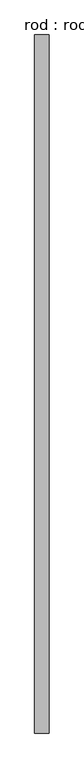
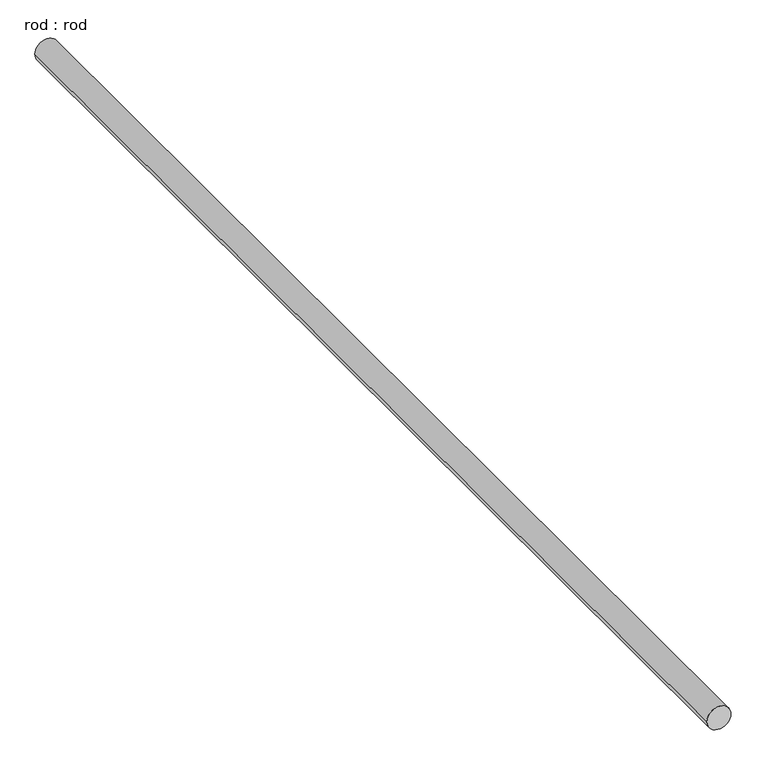
"""IFC4 building model written with IfcOpenShell, lengths in millimetres: proxy geometry, rod : rod."""

from ifc_helpers import new_model, si_unit, point, frame, frame_2d, origin, place, context, project, spatial, circle_curve, trimmed, segment, composite_curve, outline, extrude, source, transform, mapped, element, save


def rod_rod_59d15632(model_context):
    return source(origin(), model_context, "Body", "SweptSolid", [
        extrude(outline(composite_curve([segment(trimmed(circle_curve(frame_2d((0.0108462, 0.0)), 200.0), [point((0.0108462, 200.0))], [point((0.0108462, -200.0))], False, "CARTESIAN"), True, "CONTINUOUS"), segment(trimmed(circle_curve(frame_2d((0.0108462, 0.0)), 200.0), [point((0.0108462, -200.0))], [point((0.0108462, 200.0))], False, "CARTESIAN"), True, "CONTINUOUS")], self_intersect=False)), frame((0.0, -5621.5570989, 0.0), z_axis=(0.0, 1.0, 0.0), x_axis=(0.0, 0.0, 1.0)), (0.0, 0.0, 1.0), 19428.5714286),
    ])


if __name__ == "__main__":
    model = new_model("IFC4")
    model_context = context("Model", 3, world=origin())
    ifc_project = project(units=[si_unit("LENGTHUNIT", "METRE", prefix="MILLI")], contexts=[model_context])
    site = spatial("IfcSite", under=ifc_project)
    building = spatial("IfcBuilding", under=site)
    placement = place(None, origin())
    rod_rod_shape = rod_rod_59d15632(model_context)
    element("IfcBuildingElementProxy", 1, Name="rod : rod", ObjectType="rod : rod", at=placement, inside=building, context=model_context, shape_type="MappedRepresentation", body=[
        mapped(rod_rod_shape, transform((0.0, 0.0, 0.0), x_axis=(1.0, 0.0, 0.0), y_axis=(0.0, 1.0, 0.0), z_axis=(0.0, 0.0, 1.0))),
    ])
    save(model, "model.ifc")

# Revit data of these elements
# Type "rod : rod"
#   Default Elevation = 0
